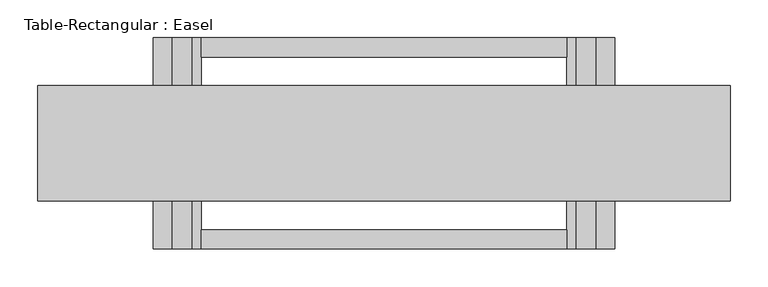
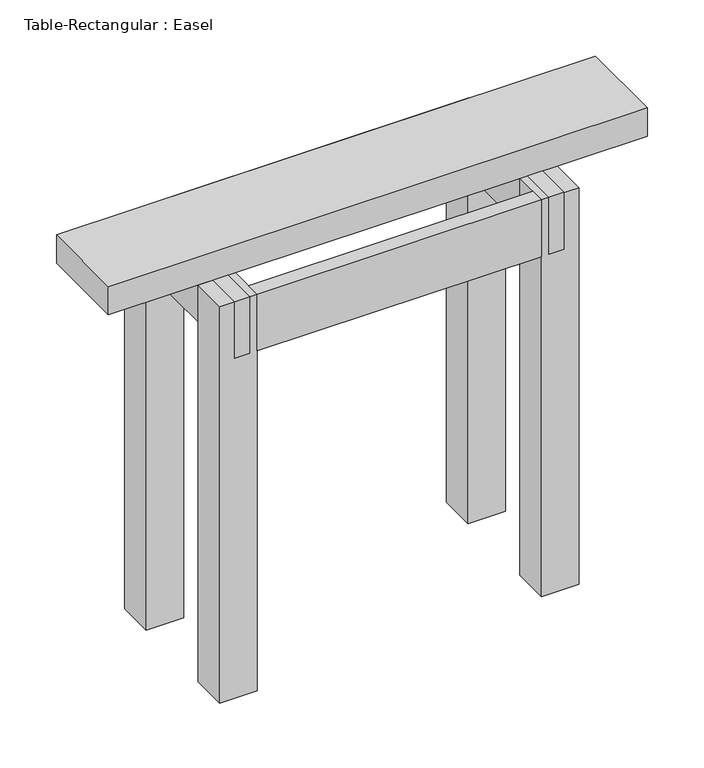
"""IFC4 building model written with IfcOpenShell, lengths in millimetres: furniture geometry, Table-Rectangular : Easel."""

from ifc_helpers import new_model, si_unit, frame, origin, origin_with_axes, place, context, project, spatial, polyline, outline, extrude, source, transform, mapped, element, save


def table_rectangular_easel_1af13968(model_context):
    return source(origin(), model_context, "Body", "SweptSolid", [
        extrude(outline(polyline([(241.3, -114.3), (241.3, -139.7), (-241.3, -139.7), (-241.3, -114.3), (241.3, -114.3)])), frame((0.0, 0.0, 609.6), z_axis=(0.0, 0.0, 1.0), x_axis=(1.0, 0.0, 0.0)), (0.0, 0.0, 1.0), 101.6),
        extrude(outline(polyline([(241.3, 114.3), (-241.3, 114.3), (-241.3, 139.7), (241.3, 139.7), (241.3, 114.3)])), frame((0.0, 0.0, 609.6), z_axis=(0.0, 0.0, 1.0), x_axis=(1.0, 0.0, 0.0)), (0.0, 0.0, 1.0), 101.6),
        extrude(outline(polyline([(-254.0, 139.7), (-254.0, -139.7), (-279.4, -139.7), (-279.4, 139.7), (-254.0, 139.7)])), frame((0.0, 0.0, 609.6), z_axis=(0.0, 0.0, 1.0), x_axis=(1.0, 0.0, 0.0)), (0.0, 0.0, 1.0), 101.6),
        extrude(outline(polyline([(254.0, 139.7), (279.4, 139.7), (279.4, -139.7), (254.0, -139.7), (254.0, 139.7)])), frame((0.0, 0.0, 609.6), z_axis=(0.0, 0.0, 1.0), x_axis=(1.0, 0.0, 0.0)), (0.0, 0.0, 1.0), 101.6),
        extrude(outline(polyline([(457.2, 76.2), (457.2, -76.2), (-457.2, -76.2), (-457.2, 76.2), (457.2, 76.2)])), frame((0.0, 0.0, 711.2), z_axis=(0.0, 0.0, 1.0), x_axis=(1.0, 0.0, 0.0)), (0.0, 0.0, 1.0), 50.8),
        extrude(outline(polyline([(-241.3, -76.2), (-241.3, -139.7), (-304.8, -139.7), (-304.8, -76.2), (-241.3, -76.2)])), origin_with_axes(), (0.0, 0.0, 1.0), 711.2),
        extrude(outline(polyline([(241.3, -76.2), (304.8, -76.2), (304.8, -139.7), (241.3, -139.7), (241.3, -76.2)])), origin_with_axes(), (0.0, 0.0, 1.0), 711.2),
        extrude(outline(polyline([(-241.3, 76.2), (-304.8, 76.2), (-304.8, 139.7), (-241.3, 139.7), (-241.3, 76.2)])), origin_with_axes(), (0.0, 0.0, 1.0), 711.2),
        extrude(outline(polyline([(241.3, 76.2), (241.3, 139.7), (304.8, 139.7), (304.8, 76.2), (241.3, 76.2)])), origin_with_axes(), (0.0, 0.0, 1.0), 711.2),
    ])


if __name__ == "__main__":
    model = new_model("IFC4")
    model_context = context("Model", 3, world=origin())
    ifc_project = project(units=[si_unit("LENGTHUNIT", "METRE", prefix="MILLI")], contexts=[model_context])
    site = spatial("IfcSite", under=ifc_project)
    building = spatial("IfcBuilding", under=site)
    placement = place(None, origin())
    table_rectangular_easel_shape = table_rectangular_easel_1af13968(model_context)
    element("IfcFurniture", 1, ObjectType="Table-Rectangular : Easel", at=placement, inside=building, context=model_context, shape_type="MappedRepresentation", body=[
        mapped(table_rectangular_easel_shape, transform((0.0, 0.0, 0.0), x_axis=(1.0, 0.0, 0.0), y_axis=(0.0, 1.0, 0.0), z_axis=(0.0, 0.0, 1.0))),
    ])
    save(model, "model.ifc")

# Revit data of these elements
# Type "Table-Rectangular : Easel"
#   Assembly Code = "E2020200"
#   Height = 2' - 6"
#   Length = 3' - 0"
#   Width = 0' - 6"
#   Base Material = Wood - Birch
#   Top Material = Wood - Birch
#   Default Elevation = 0
# Element 1 (IfcFurniture, "Table-Rectangular : Easel")
#   Materials on its faces: "Wood - Birch"
# Materials
#   "Wood - Birch": class "Unassigned", colour RGB 224 178 126, transparency 0
